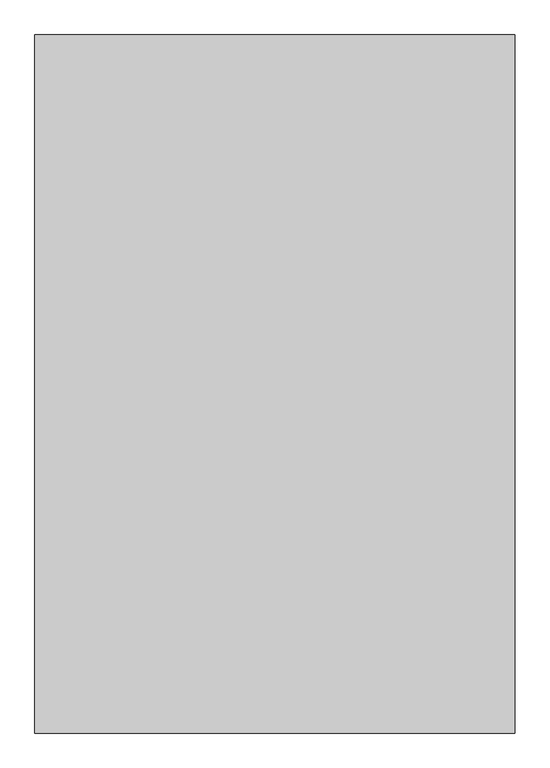
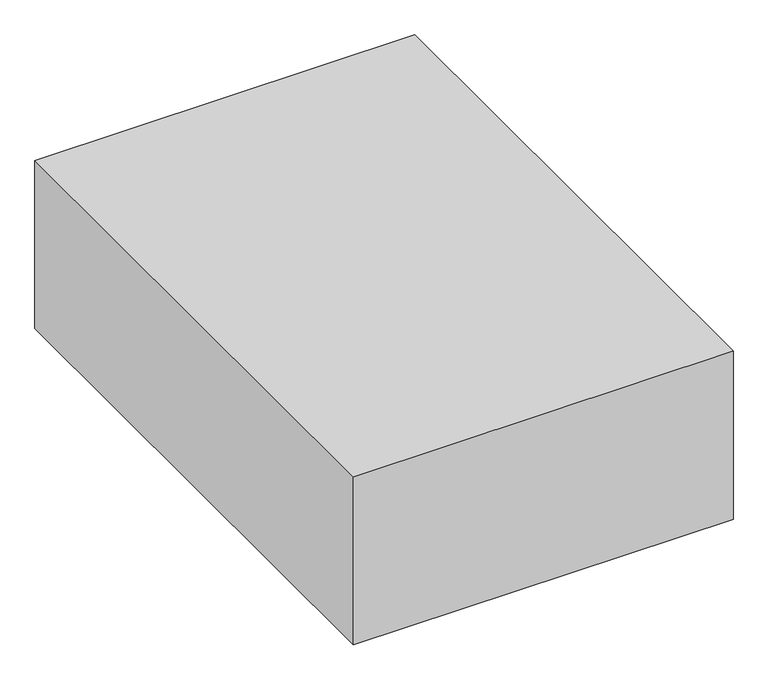
"""IFC4 building model written with IfcOpenShell, lengths in millimetres: proxy geometry, Space Planning Box_hec : Space Planning Box_hec."""

import ifcopenshell
import ifcopenshell.guid

model = None  # the IFC model being written
_history = None  # IfcOwnerHistory: only IFC2X3 demands one
_inside = {}  # id of a spatial element -> (the spatial element, [elements in it])
_under = {}  # id of a project, library or spatial element -> (it, [spatial elements below it])
_declared = {}  # id of a project -> (the project, [libraries it declares])
_typed = {}  # id of a type object -> (the type object, [elements of that type])
_made_of = {}  # id of a material, layer set ... -> (it, [elements and type objects made of it])


def new_model(schema):
    """Start an empty IFC model of exactly this schema.

    Asked for "IFC4X3", IfcOpenShell would pick the latest addendum, in which some entities
    have other attributes; the version numbers below select the first issue.
    IFC2X3 requires an IfcOwnerHistory on every rooted entity: one is made here for all.
    """
    global model, _history
    if schema == "IFC4X3":
        model = ifcopenshell.file(schema_version=(4, 3, 0, 0))
    else:
        model = ifcopenshell.file(schema=schema)
    _inside.clear()
    _under.clear()
    _declared.clear()
    _typed.clear()
    _made_of.clear()
    _history = None
    if model.schema == "IFC2X3":
        org = make("IfcOrganization", Name="unknown")
        user = make(
            "IfcPersonAndOrganization",
            ThePerson=make("IfcPerson", FamilyName="unknown"),
            TheOrganization=org,
        )
        app = make(
            "IfcApplication",
            ApplicationDeveloper=org,
            Version="unknown",
            ApplicationFullName="unknown",
            ApplicationIdentifier="unknown",
        )
        _history = make(
            "IfcOwnerHistory",
            OwningUser=user,
            OwningApplication=app,
            ChangeAction="ADDED",
            CreationDate=0,
        )
    return model


def make(cls, **values):
    """One entity of the class cls with the attributes given. An attribute that is None is left unset."""
    return model.create_entity(
        cls, **{name: value for name, value in values.items() if value is not None}
    )


def rooted(cls, **values):
    """An entity with a GlobalId (a new one), such as an element, a storey or a relation."""
    return make(cls, GlobalId=ifcopenshell.guid.new(), OwnerHistory=_history, **values)


def si_unit(unit_type, name, prefix=None):
    """IfcSIUnit, for example si_unit("LENGTHUNIT", "METRE", prefix="MILLI")."""
    return make("IfcSIUnit", UnitType=unit_type, Prefix=prefix, Name=name)


def assignment(units):
    """IfcUnitAssignment: the units of a project."""
    return None if units is None else make("IfcUnitAssignment", Units=units)


def point(xyz):
    """IfcCartesianPoint."""
    return None if xyz is None else make("IfcCartesianPoint", Coordinates=xyz)


def direction(xyz):
    """IfcDirection."""
    return None if xyz is None else make("IfcDirection", DirectionRatios=xyz)


def frame(location, z_axis=None, x_axis=None):
    """IfcAxis2Placement3D, a coordinate frame: its origin and axes. An axis left out is left unset."""
    return make(
        "IfcAxis2Placement3D",
        Location=point(location),
        Axis=direction(z_axis),
        RefDirection=direction(x_axis),
    )


def origin():
    """The frame at (0, 0, 0) with its axes left unset."""
    return frame((0.0, 0.0, 0.0))


def origin_with_axes():
    """The frame at (0, 0, 0) with the z axis (0, 0, 1) and the x axis (1, 0, 0) written out."""
    return frame((0.0, 0.0, 0.0), z_axis=(0.0, 0.0, 1.0), x_axis=(1.0, 0.0, 0.0))


def place(relative_to, where):
    """IfcLocalPlacement: puts the frame where relative to a parent placement (None: the world)."""
    return make(
        "IfcLocalPlacement", PlacementRelTo=relative_to, RelativePlacement=where
    )


def context(
    kind, dimensions, precision=None, world=None, true_north=None, identifier=None
):
    """IfcGeometricRepresentationContext, for example the 3D "Model" context."""
    return make(
        "IfcGeometricRepresentationContext",
        ContextIdentifier=identifier,
        ContextType=kind,
        CoordinateSpaceDimension=dimensions,
        Precision=precision,
        WorldCoordinateSystem=world,
        TrueNorth=true_north,
    )


def project(units=None, contexts=None):
    """IfcProject with its units and contexts."""
    return rooted(
        "IfcProject",
        Name="project",
        RepresentationContexts=contexts,
        UnitsInContext=assignment(units),
    )


def spatial(cls, under=None, at=None, **own):
    """A site, building, storey or space (cls), placed at a placement, below another one or the project."""
    s = rooted(cls, ObjectPlacement=at, **own)
    if under is not None:
        _under.setdefault(under.id(), (under, []))[1].append(s)
    return s


def polyline(points):
    """IfcPolyline through the points."""
    return make("IfcPolyline", Points=[point(p) for p in points])


def outline(outer, holes=None, kind="AREA"):
    """IfcArbitraryClosedProfileDef: a profile drawn as a closed curve; with holes, ...WithVoids."""
    if holes is None:
        return make("IfcArbitraryClosedProfileDef", ProfileType=kind, OuterCurve=outer)
    return make(
        "IfcArbitraryProfileDefWithVoids",
        ProfileType=kind,
        OuterCurve=outer,
        InnerCurves=holes,
    )


def extrude(swept, where, along, depth):
    """IfcExtrudedAreaSolid: the profile swept, set in the frame where, extruded along a direction by depth."""
    return make(
        "IfcExtrudedAreaSolid",
        SweptArea=swept,
        Position=where,
        ExtrudedDirection=direction(along),
        Depth=depth,
    )


def shape(context_of_items, identifier, shape_type, items):
    """IfcShapeRepresentation: the items that make up one representation, for example the "Body"."""
    return make(
        "IfcShapeRepresentation",
        ContextOfItems=context_of_items,
        RepresentationIdentifier=identifier,
        RepresentationType=shape_type,
        Items=items,
    )


def source(mapping_origin, context_of_items, identifier, shape_type, items):
    """IfcRepresentationMap: a shape defined once, which mapped items show again and again."""
    return make(
        "IfcRepresentationMap",
        MappingOrigin=mapping_origin,
        MappedRepresentation=shape(context_of_items, identifier, shape_type, items),
    )


def transform(
    local_origin,
    x_axis=None,
    y_axis=None,
    z_axis=None,
    scale=None,
    scale2=None,
    scale3=None,
    uniform=True,
):
    """IfcCartesianTransformationOperator3D, or its non-uniform kind. x_axis, y_axis, z_axis: its Axis1, 2, 3."""
    if uniform:
        return make(
            "IfcCartesianTransformationOperator3D",
            Axis1=direction(x_axis),
            Axis2=direction(y_axis),
            LocalOrigin=point(local_origin),
            Scale=scale,
            Axis3=direction(z_axis),
        )
    return make(
        "IfcCartesianTransformationOperator3DnonUniform",
        Axis1=direction(x_axis),
        Axis2=direction(y_axis),
        LocalOrigin=point(local_origin),
        Scale=scale,
        Axis3=direction(z_axis),
        Scale2=scale2,
        Scale3=scale3,
    )


def mapped(mapping_source, mapping_target):
    """IfcMappedItem: shows the shape of a source again, moved by a transform."""
    return make(
        "IfcMappedItem", MappingSource=mapping_source, MappingTarget=mapping_target
    )


def made_of(thing, what):
    """Note that an element or type object is made of a material, layer set ...; save() writes the relation."""
    if what is not None:
        _made_of.setdefault(what.id(), (what, []))[1].append(thing)
    return thing


def element(
    cls,
    number,
    at=None,
    inside=None,
    cuts=None,
    type_object=None,
    material=None,
    context=None,
    identifier="Body",
    shape_type=None,
    held_by="IfcProductDefinitionShape",
    body=None,
    shapes=None,
    **own,
):
    """One element of the class cls, such as IfcWall. Its Tag is "e" and its number.

    at: its placement. inside: the storey or other place that contains it. cuts: it is an
    opening in that element (IfcRelVoidsElement). A single representation is given by context,
    identifier, shape_type and body (its items); several are given by shapes. held_by: the class
    of the entity that holds the representations. save() writes the other relations.
    """
    e = rooted(cls, Tag="e%d" % number, ObjectPlacement=at, **own)
    if body is not None:
        shapes = [shape(context, identifier, shape_type, body)]
    if shapes is not None:
        e.Representation = make(held_by, Representations=shapes)
    if inside is not None:
        _inside.setdefault(inside.id(), (inside, []))[1].append(e)
    if cuts is not None:
        rooted(
            "IfcRelVoidsElement", RelatingBuildingElement=cuts, RelatedOpeningElement=e
        )
    if type_object is not None:
        _typed.setdefault(type_object.id(), (type_object, []))[1].append(e)
    return made_of(e, material)


def aggregate(whole, parts):
    """IfcRelAggregates: a whole, such as a stair, and the parts it consists of."""
    return rooted("IfcRelAggregates", RelatingObject=whole, RelatedObjects=parts)


def save(model, path):
    """Write the relations noted so far, then the file.

    IfcRelAggregates (storeys below a building ...), IfcRelContainedInSpatialStructure (elements
    in a storey), IfcRelDefinesByType, IfcRelAssociatesMaterial and IfcRelDeclares: one each for
    every whole, place, type object, material and project.
    """
    for whole, parts in _under.values():
        aggregate(whole, parts)
    for where, things in _inside.values():
        rooted(
            "IfcRelContainedInSpatialStructure",
            RelatedElements=things,
            RelatingStructure=where,
        )
    for kind, things in _typed.values():
        rooted("IfcRelDefinesByType", RelatedObjects=things, RelatingType=kind)
    for what, things in _made_of.values():
        rooted("IfcRelAssociatesMaterial", RelatedObjects=things, RelatingMaterial=what)
    for by, libraries in _declared.values():
        rooted("IfcRelDeclares", RelatingContext=by, RelatedDefinitions=libraries)
    model.write(path)


def generic_models_21711933(model_context):
    return source(origin(), model_context, "Body", "SweptSolid", [
        extrude(outline(polyline([(6400.0, 9300.0), (6400.0, -9300.0), (-6400.0, -9300.0), (-6400.0, 9300.0), (6400.0, 9300.0)])), origin_with_axes(), (0.0, 0.0, 1.0), 6000.0),
    ])


if __name__ == "__main__":
    model = new_model("IFC4")
    model_context = context("Model", 3, world=origin())
    ifc_project = project(units=[si_unit("LENGTHUNIT", "METRE", prefix="MILLI")], contexts=[model_context])
    site = spatial("IfcSite", under=ifc_project)
    building = spatial("IfcBuilding", under=site)
    placement = place(None, origin())
    generic_models_shape = generic_models_21711933(model_context)
    element("IfcBuildingElementProxy", 1, Name="Space Planning Box_hec : Space Planning Box_hec", ObjectType="Space Planning Box_hec : Space Planning Box_hec", at=placement, inside=building, context=model_context, shape_type="MappedRepresentation", body=[
        mapped(generic_models_shape, transform((0.0, 0.0, 0.0), x_axis=(1.0, 0.0, 0.0), y_axis=(0.0, 1.0, 0.0), z_axis=(0.0, 0.0, 1.0))),
    ])
    save(model, "model.ifc")

# Revit data of these elements
# Project information
#   Building Name = "MAIN GATE SECURITY BUILDING"
#   Project Status = "Project Status"
#   Client Name = "현대엔지니어링"
#   Project Address = "서울시 종로구 율곡로 75(계동)"
#   Project Name = "Therma Visayas Energy Project"
#   Project Number = "-"
# Type "Space Planning Box_hec : Space Planning Box_hec"
#   Type Comments = "..."
#   Room Name [instance default] = "?"
#   Interior Finish [instance default] = ""
#   Exterior Finish [instance default] = ""
#   Department [instance default] = ""
#   Assembly Code = "..."
#   Width [instance default] = 1524 mm
#   Program Area [instance default] = 0.00 m²
#   Length [instance default] = 1524 mm
#   Height [instance default] = 1524 mm
#   Area [instance default] = 2.32258 m²
#   Fill Color [instance default] = Cyan
#   Default Elevation = 0
# Element 1 (IfcBuildingElementProxy, "Space Planning Box_hec : Space Planning Box_hec")
#   Room Name = "Electrical Room"
#   Interior Finish = "IF1"
#   Exterior Finish = "EF1"
#   Department = "EL"
#   Width = 12800 mm
#   Program Area = 238.08 m²
#   Length = 18600 mm
#   Height = 6000 mm
#   Area = 238.08 m²
#   Fill Color = Blue
#   Materials on its faces: "Blue"
# Materials
#   "Cyan": class "Generic", colour RGB 0 255 255, transparency 0.2, Cost = 0
#   "Blue": class "Generic", colour RGB 0 0 255, transparency 0.2, Cost = 0
